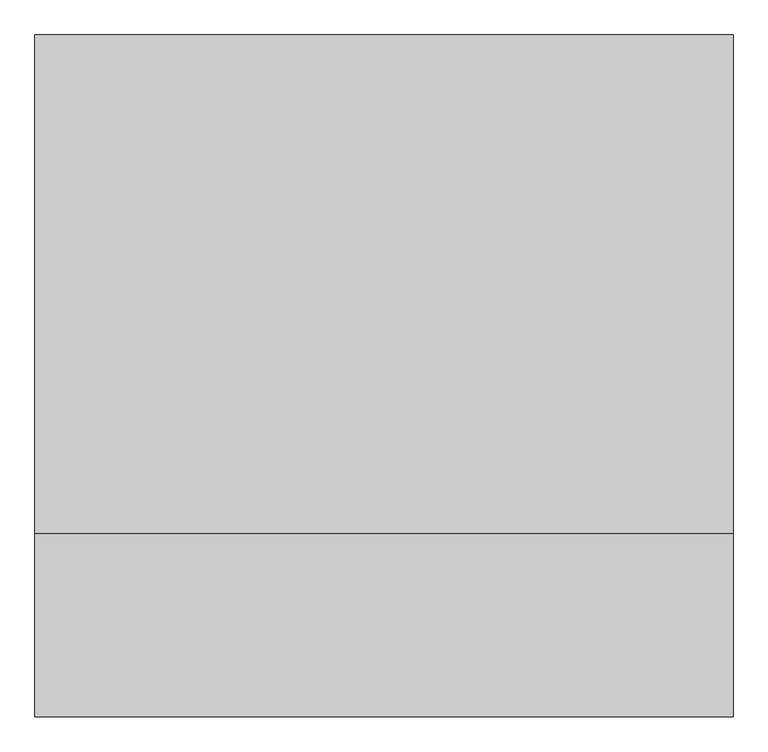
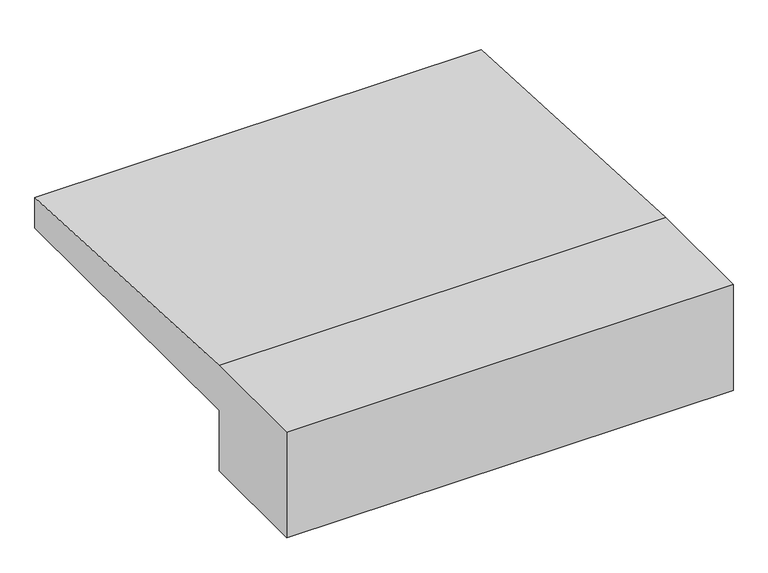
"""IFC4 building model written with IfcOpenShell, lengths in millimetres: plate geometry, 캐노피 : 캐노피."""

import ifcopenshell
import ifcopenshell.guid

model = None  # the IFC model being written
_history = None  # IfcOwnerHistory: only IFC2X3 demands one
_inside = {}  # id of a spatial element -> (the spatial element, [elements in it])
_under = {}  # id of a project, library or spatial element -> (it, [spatial elements below it])
_declared = {}  # id of a project -> (the project, [libraries it declares])
_typed = {}  # id of a type object -> (the type object, [elements of that type])
_made_of = {}  # id of a material, layer set ... -> (it, [elements and type objects made of it])


def new_model(schema):
    """Start an empty IFC model of exactly this schema.

    Asked for "IFC4X3", IfcOpenShell would pick the latest addendum, in which some entities
    have other attributes; the version numbers below select the first issue.
    IFC2X3 requires an IfcOwnerHistory on every rooted entity: one is made here for all.
    """
    global model, _history
    if schema == "IFC4X3":
        model = ifcopenshell.file(schema_version=(4, 3, 0, 0))
    else:
        model = ifcopenshell.file(schema=schema)
    _inside.clear()
    _under.clear()
    _declared.clear()
    _typed.clear()
    _made_of.clear()
    _history = None
    if model.schema == "IFC2X3":
        org = make("IfcOrganization", Name="unknown")
        user = make(
            "IfcPersonAndOrganization",
            ThePerson=make("IfcPerson", FamilyName="unknown"),
            TheOrganization=org,
        )
        app = make(
            "IfcApplication",
            ApplicationDeveloper=org,
            Version="unknown",
            ApplicationFullName="unknown",
            ApplicationIdentifier="unknown",
        )
        _history = make(
            "IfcOwnerHistory",
            OwningUser=user,
            OwningApplication=app,
            ChangeAction="ADDED",
            CreationDate=0,
        )
    return model


def make(cls, **values):
    """One entity of the class cls with the attributes given. An attribute that is None is left unset."""
    return model.create_entity(
        cls, **{name: value for name, value in values.items() if value is not None}
    )


def rooted(cls, **values):
    """An entity with a GlobalId (a new one), such as an element, a storey or a relation."""
    return make(cls, GlobalId=ifcopenshell.guid.new(), OwnerHistory=_history, **values)


def si_unit(unit_type, name, prefix=None):
    """IfcSIUnit, for example si_unit("LENGTHUNIT", "METRE", prefix="MILLI")."""
    return make("IfcSIUnit", UnitType=unit_type, Prefix=prefix, Name=name)


def assignment(units):
    """IfcUnitAssignment: the units of a project."""
    return None if units is None else make("IfcUnitAssignment", Units=units)


def point(xyz):
    """IfcCartesianPoint."""
    return None if xyz is None else make("IfcCartesianPoint", Coordinates=xyz)


def direction(xyz):
    """IfcDirection."""
    return None if xyz is None else make("IfcDirection", DirectionRatios=xyz)


def frame(location, z_axis=None, x_axis=None):
    """IfcAxis2Placement3D, a coordinate frame: its origin and axes. An axis left out is left unset."""
    return make(
        "IfcAxis2Placement3D",
        Location=point(location),
        Axis=direction(z_axis),
        RefDirection=direction(x_axis),
    )


def origin():
    """The frame at (0, 0, 0) with its axes left unset."""
    return frame((0.0, 0.0, 0.0))


def place(relative_to, where):
    """IfcLocalPlacement: puts the frame where relative to a parent placement (None: the world)."""
    return make(
        "IfcLocalPlacement", PlacementRelTo=relative_to, RelativePlacement=where
    )


def context(
    kind, dimensions, precision=None, world=None, true_north=None, identifier=None
):
    """IfcGeometricRepresentationContext, for example the 3D "Model" context."""
    return make(
        "IfcGeometricRepresentationContext",
        ContextIdentifier=identifier,
        ContextType=kind,
        CoordinateSpaceDimension=dimensions,
        Precision=precision,
        WorldCoordinateSystem=world,
        TrueNorth=true_north,
    )


def project(units=None, contexts=None):
    """IfcProject with its units and contexts."""
    return rooted(
        "IfcProject",
        Name="project",
        RepresentationContexts=contexts,
        UnitsInContext=assignment(units),
    )


def spatial(cls, under=None, at=None, **own):
    """A site, building, storey or space (cls), placed at a placement, below another one or the project."""
    s = rooted(cls, ObjectPlacement=at, **own)
    if under is not None:
        _under.setdefault(under.id(), (under, []))[1].append(s)
    return s


def polyline(points):
    """IfcPolyline through the points."""
    return make("IfcPolyline", Points=[point(p) for p in points])


def outline(outer, holes=None, kind="AREA"):
    """IfcArbitraryClosedProfileDef: a profile drawn as a closed curve; with holes, ...WithVoids."""
    if holes is None:
        return make("IfcArbitraryClosedProfileDef", ProfileType=kind, OuterCurve=outer)
    return make(
        "IfcArbitraryProfileDefWithVoids",
        ProfileType=kind,
        OuterCurve=outer,
        InnerCurves=holes,
    )


def extrude(swept, where, along, depth):
    """IfcExtrudedAreaSolid: the profile swept, set in the frame where, extruded along a direction by depth."""
    return make(
        "IfcExtrudedAreaSolid",
        SweptArea=swept,
        Position=where,
        ExtrudedDirection=direction(along),
        Depth=depth,
    )


def shape(context_of_items, identifier, shape_type, items):
    """IfcShapeRepresentation: the items that make up one representation, for example the "Body"."""
    return make(
        "IfcShapeRepresentation",
        ContextOfItems=context_of_items,
        RepresentationIdentifier=identifier,
        RepresentationType=shape_type,
        Items=items,
    )


def source(mapping_origin, context_of_items, identifier, shape_type, items):
    """IfcRepresentationMap: a shape defined once, which mapped items show again and again."""
    return make(
        "IfcRepresentationMap",
        MappingOrigin=mapping_origin,
        MappedRepresentation=shape(context_of_items, identifier, shape_type, items),
    )


def transform(
    local_origin,
    x_axis=None,
    y_axis=None,
    z_axis=None,
    scale=None,
    scale2=None,
    scale3=None,
    uniform=True,
):
    """IfcCartesianTransformationOperator3D, or its non-uniform kind. x_axis, y_axis, z_axis: its Axis1, 2, 3."""
    if uniform:
        return make(
            "IfcCartesianTransformationOperator3D",
            Axis1=direction(x_axis),
            Axis2=direction(y_axis),
            LocalOrigin=point(local_origin),
            Scale=scale,
            Axis3=direction(z_axis),
        )
    return make(
        "IfcCartesianTransformationOperator3DnonUniform",
        Axis1=direction(x_axis),
        Axis2=direction(y_axis),
        LocalOrigin=point(local_origin),
        Scale=scale,
        Axis3=direction(z_axis),
        Scale2=scale2,
        Scale3=scale3,
    )


def mapped(mapping_source, mapping_target):
    """IfcMappedItem: shows the shape of a source again, moved by a transform."""
    return make(
        "IfcMappedItem", MappingSource=mapping_source, MappingTarget=mapping_target
    )


def made_of(thing, what):
    """Note that an element or type object is made of a material, layer set ...; save() writes the relation."""
    if what is not None:
        _made_of.setdefault(what.id(), (what, []))[1].append(thing)
    return thing


def element(
    cls,
    number,
    at=None,
    inside=None,
    cuts=None,
    type_object=None,
    material=None,
    context=None,
    identifier="Body",
    shape_type=None,
    held_by="IfcProductDefinitionShape",
    body=None,
    shapes=None,
    **own,
):
    """One element of the class cls, such as IfcWall. Its Tag is "e" and its number.

    at: its placement. inside: the storey or other place that contains it. cuts: it is an
    opening in that element (IfcRelVoidsElement). A single representation is given by context,
    identifier, shape_type and body (its items); several are given by shapes. held_by: the class
    of the entity that holds the representations. save() writes the other relations.
    """
    e = rooted(cls, Tag="e%d" % number, ObjectPlacement=at, **own)
    if body is not None:
        shapes = [shape(context, identifier, shape_type, body)]
    if shapes is not None:
        e.Representation = make(held_by, Representations=shapes)
    if inside is not None:
        _inside.setdefault(inside.id(), (inside, []))[1].append(e)
    if cuts is not None:
        rooted(
            "IfcRelVoidsElement", RelatingBuildingElement=cuts, RelatedOpeningElement=e
        )
    if type_object is not None:
        _typed.setdefault(type_object.id(), (type_object, []))[1].append(e)
    return made_of(e, material)


def aggregate(whole, parts):
    """IfcRelAggregates: a whole, such as a stair, and the parts it consists of."""
    return rooted("IfcRelAggregates", RelatingObject=whole, RelatedObjects=parts)


def save(model, path):
    """Write the relations noted so far, then the file.

    IfcRelAggregates (storeys below a building ...), IfcRelContainedInSpatialStructure (elements
    in a storey), IfcRelDefinesByType, IfcRelAssociatesMaterial and IfcRelDeclares: one each for
    every whole, place, type object, material and project.
    """
    for whole, parts in _under.values():
        aggregate(whole, parts)
    for where, things in _inside.values():
        rooted(
            "IfcRelContainedInSpatialStructure",
            RelatedElements=things,
            RelatingStructure=where,
        )
    for kind, things in _typed.values():
        rooted("IfcRelDefinesByType", RelatedObjects=things, RelatingType=kind)
    for what, things in _made_of.values():
        rooted("IfcRelAssociatesMaterial", RelatedObjects=things, RelatingMaterial=what)
    for by, libraries in _declared.values():
        rooted("IfcRelDeclares", RelatingContext=by, RelatedDefinitions=libraries)
    model.write(path)


def plate_4d130048(model_context):
    return source(origin(), model_context, "Body", "SweptSolid", [
        extrude(outline(polyline([(-183.5, 800.0), (-183.5, 1150.0), (183.5, 1150.0), (1183.5, 1100.0), (1183.5, 1000.0), (183.5, 1000.0), (183.5, 800.0), (-183.5, 800.0)])), frame((-700.0, 0.0, 0.0), z_axis=(1.0, 0.0, 0.0), x_axis=(0.0, 1.0, 0.0)), (0.0, 0.0, 1.0), 1400.0),
    ])


if __name__ == "__main__":
    model = new_model("IFC4")
    model_context = context("Model", 3, world=origin())
    ifc_project = project(units=[si_unit("LENGTHUNIT", "METRE", prefix="MILLI")], contexts=[model_context])
    site = spatial("IfcSite", under=ifc_project)
    building = spatial("IfcBuilding", under=site)
    placement = place(None, origin())
    plate_shape = plate_4d130048(model_context)
    element("IfcPlate", 1, ObjectType="캐노피 : 캐노피", at=placement, inside=building, context=model_context, shape_type="MappedRepresentation", body=[
        mapped(plate_shape, transform((0.0, 0.0, 0.0), x_axis=(1.0, 0.0, 0.0), y_axis=(0.0, 1.0, 0.0), z_axis=(0.0, 0.0, 1.0))),
    ])
    save(model, "model.ifc")

# Revit data of these elements
# Type "캐노피 : 캐노피"
#   Type Mark = "203"
#   Width = 1400 mm
#   Height = 350 mm
#   돌출길이 = 1000 mm
#   Default Sill Height = 800 mm
#   Wall Closure = (empty or 0)
